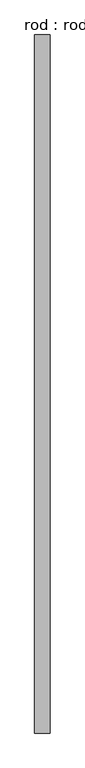
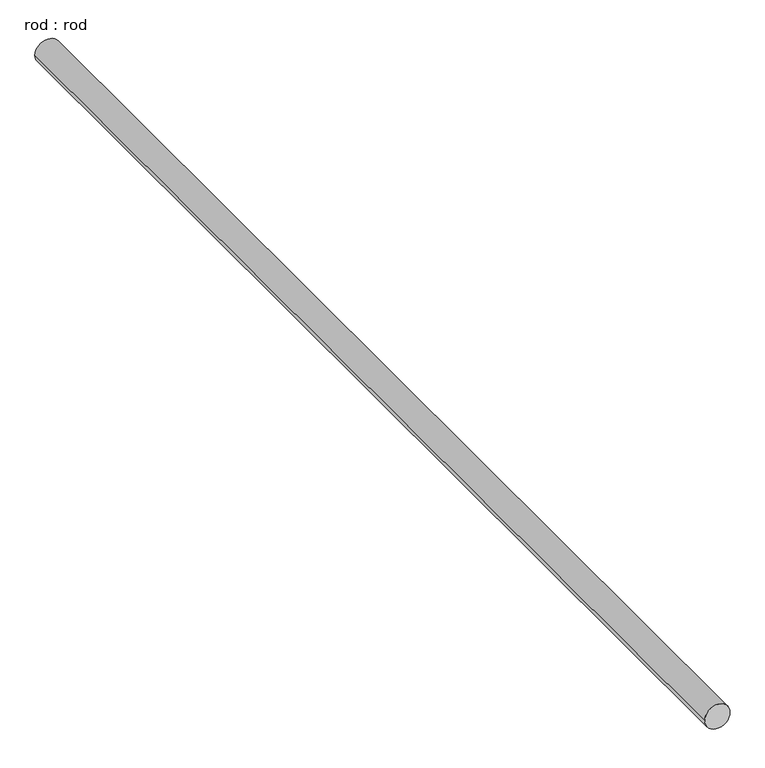
"""IFC4 building model written with IfcOpenShell, lengths in millimetres: proxy geometry, rod : rod."""

from ifc_helpers import new_model, si_unit, point, frame, frame_2d, origin, place, context, project, spatial, circle_curve, trimmed, segment, composite_curve, outline, extrude, source, transform, mapped, element, save


def rod_rod_1bf6b544(model_context):
    return source(origin(), model_context, "Body", "SweptSolid", [
        extrude(outline(composite_curve([segment(trimmed(circle_curve(frame_2d((0.0108462, 0.0)), 200.0), [point((0.0108462, 200.0))], [point((0.0108462, -200.0))], False, "CARTESIAN"), True, "CONTINUOUS"), segment(trimmed(circle_curve(frame_2d((0.0108462, 0.0)), 200.0), [point((0.0108462, -200.0))], [point((0.0108462, 200.0))], False, "CARTESIAN"), True, "CONTINUOUS")], self_intersect=False)), frame((0.0, -5067.9856704, 0.0), z_axis=(0.0, 1.0, 0.0), x_axis=(0.0, 0.0, 1.0)), (0.0, 0.0, 1.0), 18321.4285714),
    ])


if __name__ == "__main__":
    model = new_model("IFC4")
    model_context = context("Model", 3, world=origin())
    ifc_project = project(units=[si_unit("LENGTHUNIT", "METRE", prefix="MILLI")], contexts=[model_context])
    site = spatial("IfcSite", under=ifc_project)
    building = spatial("IfcBuilding", under=site)
    placement = place(None, origin())
    rod_rod_shape = rod_rod_1bf6b544(model_context)
    element("IfcBuildingElementProxy", 1, Name="rod : rod", ObjectType="rod : rod", at=placement, inside=building, context=model_context, shape_type="MappedRepresentation", body=[
        mapped(rod_rod_shape, transform((0.0, 0.0, 0.0), x_axis=(1.0, 0.0, 0.0), y_axis=(0.0, 1.0, 0.0), z_axis=(0.0, 0.0, 1.0))),
    ])
    save(model, "model.ifc")

# Revit data of these elements
# Type "rod : rod"
#   Default Elevation = 0
